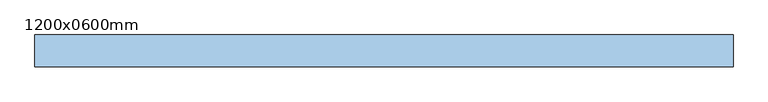
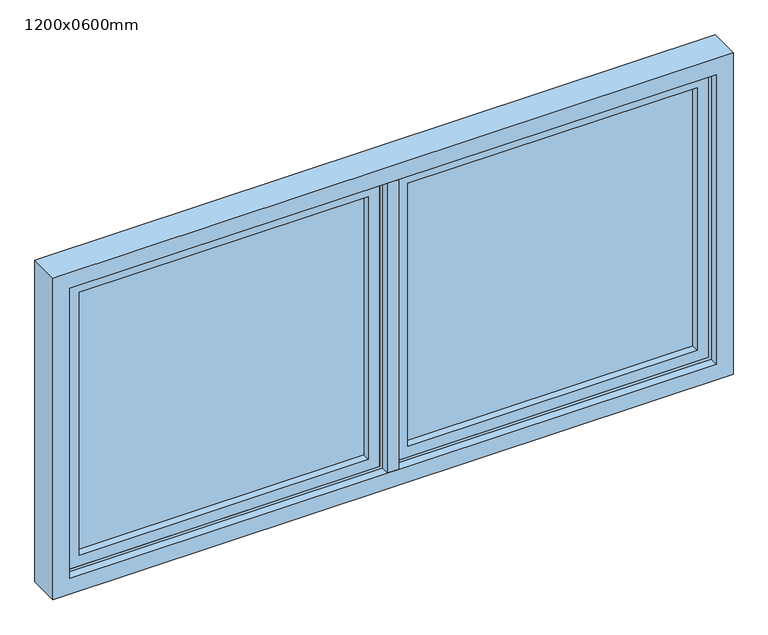
"""IFC4 building model written with IfcOpenShell, lengths in millimetres: window geometry, Janela Maxim-air - 2 Módulos : 1200x0600mm."""

from ifc_helpers import new_model, si_unit, frame, origin, place, context, project, spatial, polyline, outline, extrude, faceted_brep, source, transform, mapped, element, save


def window_1200x0600mm_366155d1(model_context):
    return source(origin(), model_context, "Body", "SolidModel", [
        extrude(outline(polyline([(552.0, -49.6), (552.0, -56.6), (28.0, -56.6), (28.0, -49.6), (552.0, -49.6)])), frame((0.0, 0.0, 1048.0), z_axis=(0.0, 0.0, 1.0), x_axis=(1.0, 0.0, 0.0)), (0.0, 0.0, 1.0), 504.0),
        faceted_brep([(35.0, -70.6, 1545.0), (35.0, -70.6, 1055.0), (35.0, -56.6, 1055.0), (35.0, -56.6, 1545.0), (28.0, -56.6, 1552.0), (28.0, -56.6, 1048.0), (28.0, -49.6, 1048.0), (28.0, -49.6, 1552.0), (35.0, -49.6, 1545.0), (35.0, -49.6, 1055.0), (35.0, -35.6, 1055.0), (35.0, -35.6, 1545.0), (15.0, -35.6, 1565.0), (15.0, -35.6, 1035.0), (15.0, -70.6, 1035.0), (15.0, -70.6, 1565.0), (545.0, -70.6, 1055.0), (545.0, -56.6, 1055.0), (552.0, -56.6, 1048.0), (552.0, -49.6, 1048.0), (545.0, -49.6, 1055.0), (545.0, -35.6, 1055.0), (565.0, -35.6, 1035.0), (565.0, -70.6, 1035.0), (545.0, -70.6, 1545.0), (545.0, -56.6, 1545.0), (552.0, -56.6, 1552.0), (552.0, -49.6, 1552.0), (545.0, -49.6, 1545.0), (545.0, -35.6, 1545.0), (565.0, -35.6, 1565.0), (565.0, -70.6, 1565.0)], [[[0, 1, 2, 3]], [[4, 5, 6, 7]], [[8, 9, 10, 11]], [[12, 13, 14, 15]], [[1, 16, 17, 2]], [[5, 18, 19, 6]], [[9, 20, 21, 10]], [[13, 22, 23, 14]], [[16, 24, 25, 17]], [[18, 26, 27, 19]], [[20, 28, 29, 21]], [[22, 30, 31, 23]], [[15, 14, 23, 31], [1, 0, 24, 16]], [[24, 0, 3, 25]], [[5, 4, 26, 18], [3, 2, 17, 25]], [[26, 4, 7, 27]], [[7, 6, 19, 27], [9, 8, 28, 20]], [[28, 8, 11, 29]], [[13, 12, 30, 22], [11, 10, 21, 29]], [[30, 12, 15, 31]]]),
        faceted_brep([(15.0, -70.6, 1565.0), (15.0, -70.6, 1035.0), (15.0, -35.6, 1035.0), (15.0, -35.6, 1565.0), (20.0, -35.6, 1560.0), (20.0, -35.6, 1040.0), (20.0, -30.6, 1040.0), (20.0, -30.6, 1560.0), (10.0, -30.6, 1570.0), (10.0, -30.6, 1030.0), (10.0, -70.6, 1030.0), (10.0, -70.6, 1570.0), (565.0, -70.6, 1035.0), (565.0, -35.6, 1035.0), (560.0, -35.6, 1040.0), (560.0, -30.6, 1040.0), (570.0, -30.6, 1030.0), (570.0, -70.6, 1030.0), (565.0, -70.6, 1565.0), (565.0, -35.6, 1565.0), (560.0, -35.6, 1560.0), (560.0, -30.6, 1560.0), (570.0, -30.6, 1570.0), (570.0, -70.6, 1570.0)], [[[0, 1, 2, 3]], [[4, 5, 6, 7]], [[8, 9, 10, 11]], [[1, 12, 13, 2]], [[5, 14, 15, 6]], [[9, 16, 17, 10]], [[12, 18, 19, 13]], [[14, 20, 21, 15]], [[16, 22, 23, 17]], [[11, 10, 17, 23], [1, 0, 18, 12]], [[18, 0, 3, 19]], [[3, 2, 13, 19], [5, 4, 20, 14]], [[20, 4, 7, 21]], [[9, 8, 22, 16], [7, 6, 15, 21]], [[22, 8, 11, 23]]]),
        extrude(outline(polyline([(-552.0, -49.6), (-28.0, -49.6), (-28.0, -56.6), (-552.0, -56.6), (-552.0, -49.6)])), frame((0.0, 0.0, 1048.0), z_axis=(0.0, 0.0, 1.0), x_axis=(1.0, 0.0, 0.0)), (0.0, 0.0, 1.0), 504.0),
        faceted_brep([(-35.0, -70.6, 1545.0), (-35.0, -56.6, 1545.0), (-35.0, -56.6, 1055.0), (-35.0, -70.6, 1055.0), (-28.0, -56.6, 1552.0), (-28.0, -49.6, 1552.0), (-28.0, -49.6, 1048.0), (-28.0, -56.6, 1048.0), (-35.0, -49.6, 1545.0), (-35.0, -35.6, 1545.0), (-35.0, -35.6, 1055.0), (-35.0, -49.6, 1055.0), (-15.0, -35.6, 1565.0), (-15.0, -70.6, 1565.0), (-15.0, -70.6, 1035.0), (-15.0, -35.6, 1035.0), (-545.0, -56.6, 1055.0), (-545.0, -70.6, 1055.0), (-552.0, -49.6, 1048.0), (-552.0, -56.6, 1048.0), (-545.0, -35.6, 1055.0), (-545.0, -49.6, 1055.0), (-565.0, -70.6, 1035.0), (-565.0, -35.6, 1035.0), (-545.0, -56.6, 1545.0), (-545.0, -70.6, 1545.0), (-552.0, -49.6, 1552.0), (-552.0, -56.6, 1552.0), (-545.0, -35.6, 1545.0), (-545.0, -49.6, 1545.0), (-565.0, -70.6, 1565.0), (-565.0, -35.6, 1565.0)], [[[0, 1, 2, 3]], [[4, 5, 6, 7]], [[8, 9, 10, 11]], [[12, 13, 14, 15]], [[3, 2, 16, 17]], [[7, 6, 18, 19]], [[11, 10, 20, 21]], [[15, 14, 22, 23]], [[17, 16, 24, 25]], [[19, 18, 26, 27]], [[21, 20, 28, 29]], [[23, 22, 30, 31]], [[13, 30, 22, 14], [3, 17, 25, 0]], [[25, 24, 1, 0]], [[7, 19, 27, 4], [1, 24, 16, 2]], [[27, 26, 5, 4]], [[5, 26, 18, 6], [11, 21, 29, 8]], [[29, 28, 9, 8]], [[15, 23, 31, 12], [9, 28, 20, 10]], [[31, 30, 13, 12]]]),
        faceted_brep([(-15.0, -70.6, 1565.0), (-15.0, -35.6, 1565.0), (-15.0, -35.6, 1035.0), (-15.0, -70.6, 1035.0), (-20.0, -35.6, 1560.0), (-20.0, -30.6, 1560.0), (-20.0, -30.6, 1040.0), (-20.0, -35.6, 1040.0), (-10.0, -30.6, 1570.0), (-10.0, -70.6, 1570.0), (-10.0, -70.6, 1030.0), (-10.0, -30.6, 1030.0), (-565.0, -35.6, 1035.0), (-565.0, -70.6, 1035.0), (-560.0, -30.6, 1040.0), (-560.0, -35.6, 1040.0), (-570.0, -70.6, 1030.0), (-570.0, -30.6, 1030.0), (-565.0, -35.6, 1565.0), (-565.0, -70.6, 1565.0), (-560.0, -30.6, 1560.0), (-560.0, -35.6, 1560.0), (-570.0, -70.6, 1570.0), (-570.0, -30.6, 1570.0)], [[[0, 1, 2, 3]], [[4, 5, 6, 7]], [[8, 9, 10, 11]], [[3, 2, 12, 13]], [[7, 6, 14, 15]], [[11, 10, 16, 17]], [[13, 12, 18, 19]], [[15, 14, 20, 21]], [[17, 16, 22, 23]], [[9, 22, 16, 10], [3, 13, 19, 0]], [[19, 18, 1, 0]], [[1, 18, 12, 2], [7, 15, 21, 4]], [[21, 20, 5, 4]], [[11, 17, 23, 8], [5, 20, 14, 6]], [[23, 22, 9, 8]]]),
        extrude(outline(polyline([(10.0, -85.6), (-10.0, -85.6), (-10.0, -30.6), (10.0, -30.6), (10.0, -85.6)])), frame((0.0, 0.0, 1030.0), z_axis=(0.0, 0.0, 1.0), x_axis=(1.0, 0.0, 0.0)), (0.0, 0.0, 1.0), 540.0),
        extrude(outline(polyline([(1600.0, 600.0), (1600.0, -600.0), (1000.0, -600.0), (1000.0, 600.0), (1600.0, 600.0)]), holes=[polyline([(1030.0, 570.0), (1030.0, -570.0), (1570.0, -570.0), (1570.0, 570.0), (1030.0, 570.0)])]), frame((0.0, -85.6, 0.0), z_axis=(0.0, 1.0, 0.0), x_axis=(0.0, 0.0, 1.0)), (0.0, 0.0, 1.0), 55.0),
    ])


if __name__ == "__main__":
    model = new_model("IFC4")
    model_context = context("Model", 3, world=origin())
    ifc_project = project(units=[si_unit("LENGTHUNIT", "METRE", prefix="MILLI")], contexts=[model_context])
    site = spatial("IfcSite", under=ifc_project)
    building = spatial("IfcBuilding", under=site)
    placement = place(None, origin())
    window_1200x0600mm_shape = window_1200x0600mm_366155d1(model_context)
    element("IfcWindow", 1, ObjectType="Janela Maxim-air - 2 Módulos : 1200x0600mm", at=placement, inside=building, context=model_context, shape_type="MappedRepresentation", body=[
        mapped(window_1200x0600mm_shape, transform((0.0, 0.0, 0.0), x_axis=(1.0, 0.0, 0.0), y_axis=(0.0, 1.0, 0.0), z_axis=(0.0, 0.0, 1.0))),
    ])
    save(model, "model.ifc")

# Revit data of these elements
# Type "Janela Maxim-air - 2 Módulos : 1200x0600mm"
#   Type Mark = "J10"
#   SINAPI = ""
#   ref. vert. basc. = 54.00 cm
#   ref. horiz. basc. = 56.00 cm
#   Largura Batente = 5.50 cm
#   Height = 60.00 cm
#   Default Sill Height = 100.00 cm
#   Width = 120.00 cm
#   Material Quadro = Metal - Alumínio
#   Material Painel = Vidro
#   Wall Closure = (empty or 0)
#   Assembly Code = ""
# Element 1 (IfcWindow, "Janela Maxim-air - 2 Módulos : 1200x0600mm")
#   Materials on its faces: "Metal - Alumínio", "Vidro"
# Materials
#   "Metal - Alumínio": class "Metal", colour RGB 244 244 244, transparency 0
#   "Vidro": class "Vidro", colour RGB 230 230 230, transparency 0.75, Cost = 0
